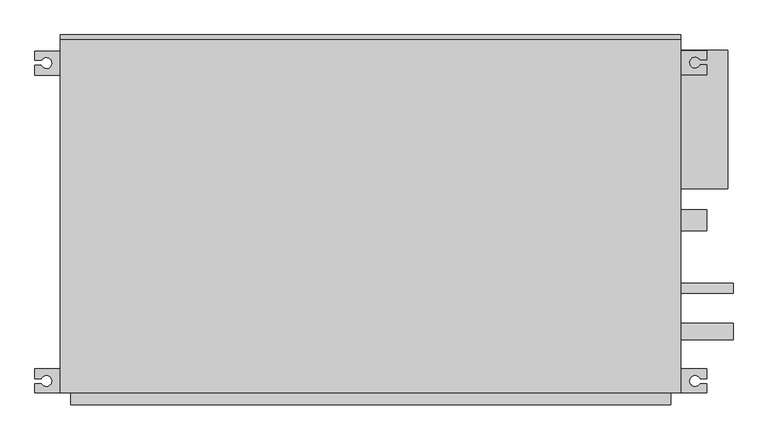
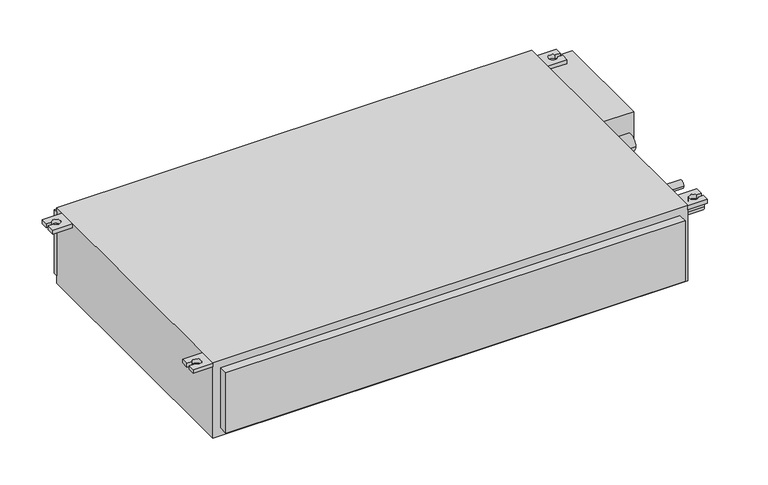
"""IFC4 building model written with IfcOpenShell, lengths in millimetres: proxy geometry, PEFY-P-NMSU-E_Low_Profile_Ducted : PEFY-P24NMSU-E."""

from ifc_helpers import new_model, si_unit, point, frame, frame_2d, origin, origin_with_axes, place, context, project, spatial, polyline, circle_curve, trimmed, segment, composite_curve, outline, extrude, source, transform, mapped, element, save


def mechanical_equipment_2ac3c092(model_context):
    return source(origin(), model_context, "Body", "SweptSolid", [
        extrude(outline(composite_curve([segment(polyline([(-644.3, 282.0), (-644.3, 300.9759165), (-632.1454311, 300.9759165)]), True, "CONTINUOUS"), segment(trimmed(circle_curve(frame_2d((-622.2863556, 305.4254582)), 10.8166442), [point((-632.1454311, 300.9759165))], [point((-631.8387803, 310.5))], True, "CARTESIAN"), True, "CONTINUOUS"), segment(polyline([(-631.8387803, 310.5), (-644.3, 310.5), (-644.3, 328.0), (-595.3, 328.0), (-595.3, 282.0), (-644.3, 282.0)]), True, "CONTINUOUS")], self_intersect=False)), frame((0.0, 0.0, 188.55), z_axis=(0.0, 0.0, 1.0), x_axis=(1.0, 0.0, 0.0)), (0.0, 0.0, 1.0), 10.0),
        extrude(outline(composite_curve([segment(polyline([(-644.3, -281.0), (-595.3, -281.0), (-595.3, -327.0), (-644.3, -327.0), (-644.3, -309.5), (-631.8387803, -309.5)]), True, "CONTINUOUS"), segment(trimmed(circle_curve(frame_2d((-622.2863556, -304.4254582)), 10.8166442), [point((-631.8387803, -309.5))], [point((-632.1454311, -299.9759165))], True, "CARTESIAN"), True, "CONTINUOUS"), segment(polyline([(-632.1454311, -299.9759165), (-644.3, -299.9759165), (-644.3, -281.0)]), True, "CONTINUOUS")], self_intersect=False)), frame((0.0, 0.0, 188.55), z_axis=(0.0, 0.0, 1.0), x_axis=(1.0, 0.0, 0.0)), (0.0, 0.0, 1.0), 10.0),
        extrude(outline(composite_curve([segment(polyline([(644.3, 282.9429009), (595.3, 282.9429009), (595.3, 328.9429009), (644.3, 328.9429009), (644.3, 311.4429009), (631.8387803, 311.4429009)]), True, "CONTINUOUS"), segment(trimmed(circle_curve(frame_2d((622.2863556, 306.3683591)), 10.8166442), [point((631.8387803, 311.4429009))], [point((632.1454311, 301.9188174))], True, "CARTESIAN"), True, "CONTINUOUS"), segment(polyline([(632.1454311, 301.9188174), (644.3, 301.9188174), (644.3, 282.9429009)]), True, "CONTINUOUS")], self_intersect=False)), frame((0.0, 0.0, 188.55), z_axis=(0.0, 0.0, 1.0), x_axis=(1.0, 0.0, 0.0)), (0.0, 0.0, 1.0), 10.0),
        extrude(outline(composite_curve([segment(polyline([(644.3, -281.0), (644.3, -299.9759165), (632.1454311, -299.9759165)]), True, "CONTINUOUS"), segment(trimmed(circle_curve(frame_2d((622.2863556, -304.4254582)), 10.8166442), [point((632.1454311, -299.9759165))], [point((631.8387803, -309.5))], True, "CARTESIAN"), True, "CONTINUOUS"), segment(polyline([(631.8387803, -309.5), (644.3, -309.5), (644.3, -327.0), (595.3, -327.0), (595.3, -281.0), (644.3, -281.0)]), True, "CONTINUOUS")], self_intersect=False)), frame((0.0, 0.0, 188.55), z_axis=(0.0, 0.0, 1.0), x_axis=(1.0, 0.0, 0.0)), (0.0, 0.0, 1.0), 10.0),
        extrude(outline(polyline([(595.3, 350.04375), (-595.3, 350.04375), (-595.3, 359.5477547), (595.3, 359.5477547), (595.3, 350.04375)])), frame((0.0, 0.0, 20.0), z_axis=(0.0, 0.0, 1.0), x_axis=(1.0, 0.0, 0.0)), (0.0, 0.0, 1.0), 168.55),
        extrude(outline(composite_curve([segment(trimmed(circle_curve(frame_2d((4.0570991, 59.8)), 20.0), [point((-15.9429009, 59.8))], [point((24.0570991, 59.8))], False, "CARTESIAN"), True, "CONTINUOUS"), segment(trimmed(circle_curve(frame_2d((4.0570991, 59.8)), 20.0), [point((24.0570991, 59.8))], [point((-15.9429009, 59.8))], False, "CARTESIAN"), True, "CONTINUOUS")], self_intersect=False)), frame((595.3, 0.0, 0.0), z_axis=(1.0, 0.0, 0.0), x_axis=(0.0, 1.0, 0.0)), (0.0, 0.0, 1.0), 26.9863556),
        extrude(outline(composite_curve([segment(trimmed(circle_curve(frame_2d((4.0570991, 149.6)), 20.0), [point((-15.9429009, 149.6))], [point((24.0570991, 149.6))], False, "CARTESIAN"), True, "CONTINUOUS"), segment(trimmed(circle_curve(frame_2d((4.0570991, 149.6)), 20.0), [point((24.0570991, 149.6))], [point((-15.9429009, 149.6))], False, "CARTESIAN"), True, "CONTINUOUS")], self_intersect=False)), frame((595.3, 0.0, 0.0), z_axis=(1.0, 0.0, 0.0), x_axis=(0.0, 1.0, 0.0)), (0.0, 0.0, 1.0), 49.0),
        extrude(outline(composite_curve([segment(trimmed(circle_curve(frame_2d((-126.5596979, 100.0)), 9.5), [point((-136.0596979, 100.0))], [point((-117.0596979, 100.0))], False, "CARTESIAN"), True, "CONTINUOUS"), segment(trimmed(circle_curve(frame_2d((-126.5596979, 100.0)), 9.5), [point((-117.0596979, 100.0))], [point((-136.0596979, 100.0))], False, "CARTESIAN"), True, "CONTINUOUS")], self_intersect=False)), frame((595.3, 0.0, 0.0), z_axis=(1.0, 0.0, 0.0), x_axis=(0.0, 1.0, 0.0)), (0.0, 0.0, 1.0), 100.0),
        extrude(outline(composite_curve([segment(trimmed(circle_curve(frame_2d((-209.7540575, 100.0)), 15.9), [point((-225.6540575, 100.0))], [point((-193.8540575, 100.0))], False, "CARTESIAN"), True, "CONTINUOUS"), segment(trimmed(circle_curve(frame_2d((-209.7540575, 100.0)), 15.9), [point((-193.8540575, 100.0))], [point((-225.6540575, 100.0))], False, "CARTESIAN"), True, "CONTINUOUS")], self_intersect=False)), frame((595.3, 0.0, 0.0), z_axis=(1.0, 0.0, 0.0), x_axis=(0.0, 1.0, 0.0)), (0.0, 0.0, 1.0), 100.0),
        extrude(outline(polyline([(685.3, 330.0), (685.3, 64.0570991), (595.3, 64.0570991), (595.3, 330.0), (685.3, 330.0)])), frame((0.0, 0.0, 20.0), z_axis=(0.0, 0.0, 1.0), x_axis=(1.0, 0.0, 0.0)), (0.0, 0.0, 1.0), 159.8),
        extrude(outline(polyline([(575.3, -350.04375), (-575.3, -350.04375), (-575.3, -327.0), (575.3, -327.0), (575.3, -350.04375)])), frame((0.0, 0.0, 20.0), z_axis=(0.0, 0.0, 1.0), x_axis=(1.0, 0.0, 0.0)), (0.0, 0.0, 1.0), 159.8),
        extrude(outline(polyline([(-595.3, -327.0), (-595.3, 350.04375), (595.3, 350.04375), (595.3, -327.0), (-595.3, -327.0)])), origin_with_axes(), (0.0, 0.0, 1.0), 200.0),
    ])


if __name__ == "__main__":
    model = new_model("IFC4")
    model_context = context("Model", 3, world=origin())
    ifc_project = project(units=[si_unit("LENGTHUNIT", "METRE", prefix="MILLI")], contexts=[model_context])
    site = spatial("IfcSite", under=ifc_project)
    building = spatial("IfcBuilding", under=site)
    placement = place(None, origin())
    mechanical_equipment_shape = mechanical_equipment_2ac3c092(model_context)
    element("IfcBuildingElementProxy", 1, Name="PEFY-P-NMSU-E_Low_Profile_Ducted : PEFY-P24NMSU-E", ObjectType="PEFY-P-NMSU-E_Low_Profile_Ducted : PEFY-P24NMSU-E", at=placement, inside=building, context=model_context, shape_type="MappedRepresentation", body=[
        mapped(mechanical_equipment_shape, transform((0.0, 0.0, 0.0), x_axis=(1.0, 0.0, 0.0), y_axis=(0.0, 1.0, 0.0), z_axis=(0.0, 0.0, 1.0))),
    ])
    save(model, "model.ifc")

# Revit data of these elements
# Type "PEFY-P-NMSU-E_Low_Profile_Ducted : PEFY-P24NMSU-E"
#   Subcategory = "HVAC"
#   Standard Air Filter = "Polypropylene Honeycomb"
#   Specification URL = "http://www.mrslim.com/customerCare/resources.asp"
#   Sound Pressure Levels (dB(A)) = "30-35-40"
#   SmartBIM Object Created By = "Reed Construction Data"
#   Refirigerant Pipe diameter (Liquid) = "3/8\""
#   Refirigerant Pipe diameter (Gas) = "5/8\""
#   Power Source = "208/230, 1, 60"
#   Power Consumption Heating = "0.10 kW"
#   Power Consumption Cooling = "0.12 kW"
#   Unit Weight (LBS) = "62"
#   Model = "PEFY-P24NMSU-E"
#   Manufacturer URL = "http://www.mrslim.com/customerCare/resources.asp"
#   Manufacturer = "Mitsubishi Electric"
#   Installation URL = "http://www.mrslim.com/customerCare/resources.asp"
#   Fan Motor Type = "DC Motor"
#   Fan Motor Output = "0.096 kW"
#   MCA = "1.57/1.73"
#   MOCP = "15 A"
#   E.S.P (In. W.G.) = ".02-.20"
#   Drainpipe Dimension = "1-1/4"
#   Description = "Ceiling Concealed Ducted Low Profile"
#   Condensate Lift Mechanism = "21-11/16\""
#   Coil Type = "Cross Fin"
#   Heating Capacity (BTU) = "27000"
#   Fan Type x Quantity = "Sirocco Fan x 2"
#   Current Heating = "0.83 A"
#   Current Cooling = "0.93 A"
#   Cooling Capacity (BTU) = "24000"
#   Fan capacity (CFM) = "423-565-706"
#   Assembly Code = "D3050200"
#   95 CSI = "15760"
#   04 CSI = "23 82 19 "
#   Width = 1190.6 mm
#   Voltage = 208 V
#   Unit Supply Airflow [instance default] = 390 CFM
#   Unit Return Airflow [instance default] = 390 CFM
#   SmartBIM Object Version = 3
#   Height = 200 mm
#   Drain Pipe Radius = 20 mm
#   Depth = 700.088 mm
#   Default Elevation = 1219.2 mm
#   C = 1288.6 mm
#   Brazing Connection Radius (Liquid) = 9.5 mm
#   Brazing Connection Radius (Gas) = 15.9 mm
#   Suspension Bolt Pitch = 1242.6 mm
#   Apparent Load = 0 VA
#   Air Outlet Width = 1150.6 mm
#   Air Inlet Width = 1190.6 mm
#   Air Outlet Height = 159.8 mm
#   Air Inlet Height = 169 mm
#   Number of Poles = 1
#   Load Classification = Other
#   External Finish = Galvanized Steel Sheet
#   Air Outlet Unit Material = Metal Grill
#   Air Inlet Unit Material = Grill
#   URL = ""
# Element 1 (IfcBuildingElementProxy, "PEFY-P-NMSU-E_Low_Profile_Ducted : PEFY-P24NMSU-E")
#   Unit Supply Airflow = 300 CFM
#   Unit Return Airflow = 0 CFM
#   Materials on its faces: "Galvanized Steel Sheet", "Grill", "Metal Grill"
# Materials
#   "Galvanized Steel Sheet": class "Metal", colour RGB 189 187 185, transparency 0
#   "Metal Grill": class "Metal", colour RGB 10 10 10, transparency 0
#   "Grill": class "Plastic", colour RGB 5 5 5, transparency 0
